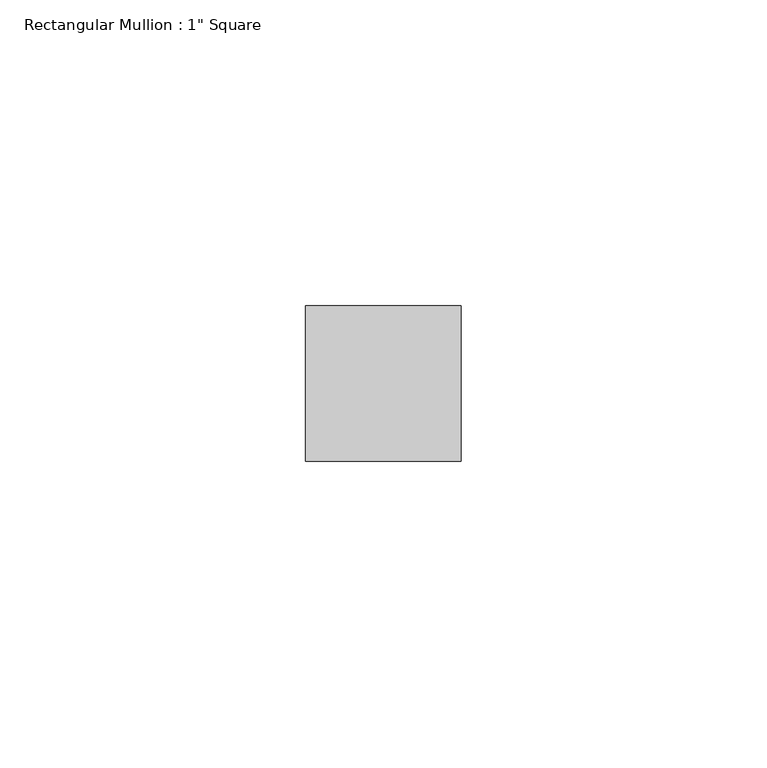
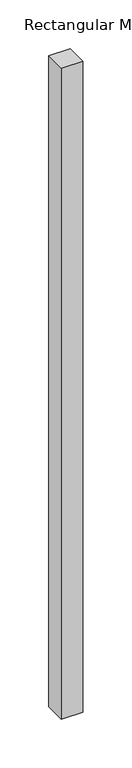
"""IFC4 building model written with IfcOpenShell, lengths in millimetres: member geometry."""

from ifc_helpers import new_model, si_unit, frame, origin, place, context, project, spatial, polyline, outline, extrude, source, transform, mapped, element, save


def member_3c836d14(model_context):
    return source(origin(), model_context, "Body", "SweptSolid", [
        extrude(outline(polyline([(0.0, 12.7), (0.0, -12.7), (-25.4, -12.7), (-25.4, 12.7), (0.0, 12.7)])), frame((0.0, 0.0, -812.8), z_axis=(0.0, 0.0, 1.0), x_axis=(1.0, 0.0, 0.0)), (0.0, 0.0, 1.0), 812.8),
    ])


if __name__ == "__main__":
    model = new_model("IFC4")
    model_context = context("Model", 3, world=origin())
    ifc_project = project(units=[si_unit("LENGTHUNIT", "METRE", prefix="MILLI")], contexts=[model_context])
    site = spatial("IfcSite", under=ifc_project)
    building = spatial("IfcBuilding", under=site)
    placement = place(None, origin())
    member_shape = member_3c836d14(model_context)
    element("IfcMember", 1, ObjectType="Rectangular Mullion : 1\" Square", at=placement, inside=building, context=model_context, shape_type="MappedRepresentation", body=[
        mapped(member_shape, transform((0.0, 0.0, 0.0), x_axis=(1.0, 0.0, 0.0), y_axis=(0.0, 1.0, 0.0), z_axis=(0.0, 0.0, 1.0))),
    ])
    save(model, "model.ifc")

# Revit data of these elements
# Type "Rectangular Mullion : 1\" Square"
#   built-in parameter 1007304 = 0.0833333 (stored number, unit not read)
#   built-in parameter 1007301 = 0.0416667 (stored number, unit not read)
#   built-in parameter 1007300 = 0.0416667 (stored number, unit not read)
# Element 1 (IfcMember, "Rectangular Mullion : 1\" Square")
#   Materials on its faces: "Metal - Aluminum"
# Materials
#   "Metal - Aluminum": class "Metal", colour RGB 247 247 247, transparency 0
